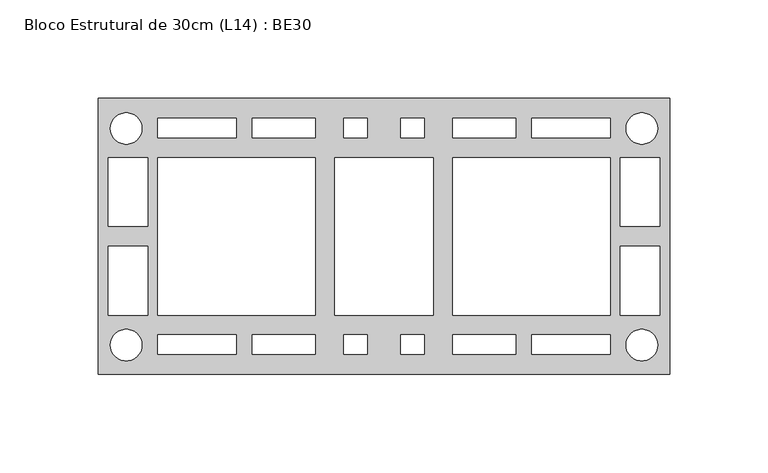
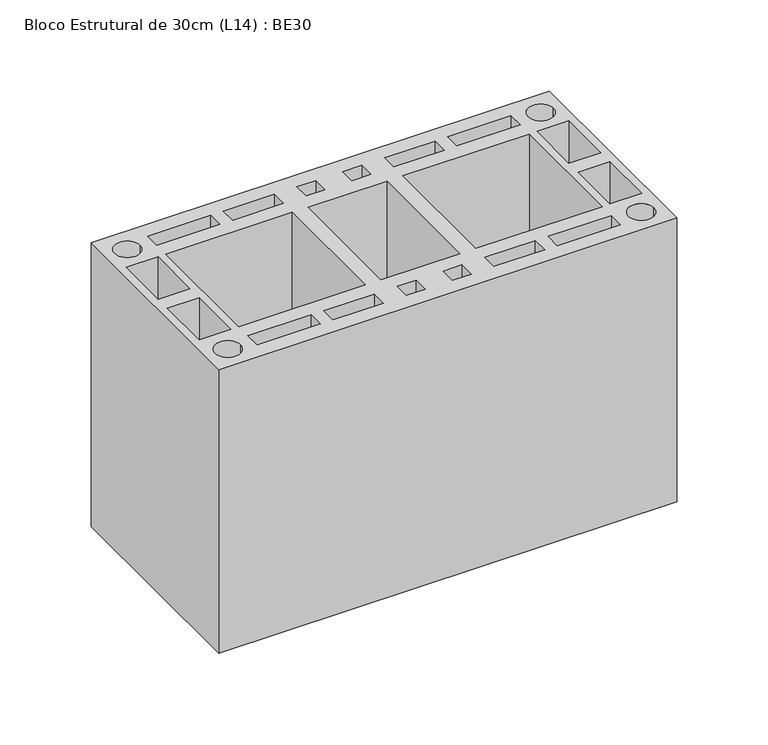
"""IFC4 building model written with IfcOpenShell, lengths in millimetres: proxy geometry, Bloco Estrutural de 30cm (L14) : BE30."""

from ifc_helpers import new_model, si_unit, point, frame_2d, origin, origin_with_axes, place, context, project, spatial, polyline, circle_curve, trimmed, segment, composite_curve, outline, extrude, source, transform, mapped, element, save


def bloco_estrutural_de_30cm_l14_be30_19b25b02(model_context):
    return source(origin(), model_context, "Body", "SweptSolid", [
        extrude(outline(polyline([(290.0, 0.0), (0.0, 0.0), (0.0, 140.0), (290.0, 140.0), (290.0, 0.0)]), holes=[composite_curve([segment(trimmed(circle_curve(frame_2d((14.1087523, 124.7509514)), 8.0), [point((6.1087523, 124.7509514))], [point((22.1087523, 124.7509514))], True, "CARTESIAN"), True, "CONTINUOUS"), segment(trimmed(circle_curve(frame_2d((14.1087523, 124.7509514)), 8.0), [point((22.1087523, 124.7509514))], [point((6.1087523, 124.7509514))], True, "CARTESIAN"), True, "CONTINUOUS")], self_intersect=False), composite_curve([segment(trimmed(circle_curve(frame_2d((14.1087523, 14.7509514)), 8.0), [point((6.1087523, 14.7509514))], [point((22.1087523, 14.7509514))], True, "CARTESIAN"), True, "CONTINUOUS"), segment(trimmed(circle_curve(frame_2d((14.1087523, 14.7509514)), 8.0), [point((22.1087523, 14.7509514))], [point((6.1087523, 14.7509514))], True, "CARTESIAN"), True, "CONTINUOUS")], self_intersect=False), polyline([(110.0, 110.0), (30.0, 110.0), (30.0, 30.0), (110.0, 30.0), (110.0, 110.0)]), polyline([(170.0, 110.0), (120.0, 110.0), (120.0, 30.0), (170.0, 30.0), (170.0, 110.0)]), polyline([(70.0, 130.0), (30.0, 130.0), (30.0, 120.0), (70.0, 120.0), (70.0, 130.0)]), polyline([(70.0, 20.0), (30.0, 20.0), (30.0, 10.0), (70.0, 10.0), (70.0, 20.0)]), polyline([(78.0, 130.0), (78.0, 120.0), (110.0, 120.0), (110.0, 130.0), (78.0, 130.0)]), polyline([(78.0, 20.0), (78.0, 10.0), (110.0, 10.0), (110.0, 20.0), (78.0, 20.0)]), composite_curve([segment(trimmed(circle_curve(frame_2d((275.8912477, 124.7509514)), 8.0), [point((283.8912477, 124.7509514))], [point((267.8912477, 124.7509514))], True, "CARTESIAN"), True, "CONTINUOUS"), segment(trimmed(circle_curve(frame_2d((275.8912477, 124.7509514)), 8.0), [point((267.8912477, 124.7509514))], [point((283.8912477, 124.7509514))], True, "CARTESIAN"), True, "CONTINUOUS")], self_intersect=False), composite_curve([segment(trimmed(circle_curve(frame_2d((275.8912477, 14.7509514)), 8.0), [point((283.8912477, 14.7509514))], [point((267.8912477, 14.7509514))], True, "CARTESIAN"), True, "CONTINUOUS"), segment(trimmed(circle_curve(frame_2d((275.8912477, 14.7509514)), 8.0), [point((267.8912477, 14.7509514))], [point((283.8912477, 14.7509514))], True, "CARTESIAN"), True, "CONTINUOUS")], self_intersect=False), polyline([(180.0, 110.0), (180.0, 30.0), (260.0, 30.0), (260.0, 110.0), (180.0, 110.0)]), polyline([(220.0, 130.0), (220.0, 120.0), (260.0, 120.0), (260.0, 130.0), (220.0, 130.0)]), polyline([(220.0, 20.0), (220.0, 10.0), (260.0, 10.0), (260.0, 20.0), (220.0, 20.0)]), polyline([(212.0, 130.0), (180.0, 130.0), (180.0, 120.0), (212.0, 120.0), (212.0, 130.0)]), polyline([(212.0, 20.0), (180.0, 20.0), (180.0, 10.0), (212.0, 10.0), (212.0, 20.0)]), polyline([(25.0, 110.0), (5.0, 110.0), (5.0, 75.0), (25.0, 75.0), (25.0, 110.0)]), polyline([(25.0, 30.0), (25.0, 65.0), (5.0, 65.0), (5.0, 30.0), (25.0, 30.0)]), polyline([(265.0, 110.0), (265.0, 75.0), (285.0, 75.0), (285.0, 110.0), (265.0, 110.0)]), polyline([(265.0, 30.0), (285.0, 30.0), (285.0, 65.0), (265.0, 65.0), (265.0, 30.0)]), polyline([(153.5, 20.0), (153.5, 10.0), (165.5, 10.0), (165.5, 20.0), (153.5, 20.0)]), polyline([(136.5, 20.0), (124.5, 20.0), (124.5, 10.0), (136.5, 10.0), (136.5, 20.0)]), polyline([(153.5, 120.0), (165.5, 120.0), (165.5, 130.0), (153.5, 130.0), (153.5, 120.0)]), polyline([(136.5, 120.0), (136.5, 130.0), (124.5, 130.0), (124.5, 120.0), (136.5, 120.0)])]), origin_with_axes(), (0.0, 0.0, 1.0), 190.0),
    ])


if __name__ == "__main__":
    model = new_model("IFC4")
    model_context = context("Model", 3, world=origin())
    ifc_project = project(units=[si_unit("LENGTHUNIT", "METRE", prefix="MILLI")], contexts=[model_context])
    site = spatial("IfcSite", under=ifc_project)
    building = spatial("IfcBuilding", under=site)
    placement = place(None, origin())
    bloco_estrutural_de_30cm_l14_be30_shape = bloco_estrutural_de_30cm_l14_be30_19b25b02(model_context)
    element("IfcBuildingElementProxy", 1, Name="Bloco Estrutural de 30cm (L14) : BE30", ObjectType="Bloco Estrutural de 30cm (L14) : BE30", at=placement, inside=building, context=model_context, shape_type="MappedRepresentation", body=[
        mapped(bloco_estrutural_de_30cm_l14_be30_shape, transform((0.0, 0.0, 0.0), x_axis=(1.0, 0.0, 0.0), y_axis=(0.0, 1.0, 0.0), z_axis=(0.0, 0.0, 1.0))),
    ])
    save(model, "model.ifc")

# Revit data of these elements
# Type "Bloco Estrutural de 30cm (L14) : BE30"
#   Material [instance default] = Blocos Cerâmicos
#   Default Elevation = 0
# Element 1 (IfcBuildingElementProxy, "Bloco Estrutural de 30cm (L14) : BE30")
#   Materials on its faces: "Blocos Cerâmicos"
# Materials
#   "Blocos Cerâmicos": class "Genérico", colour RGB 177 84 47, transparency 0, Cost = 0
